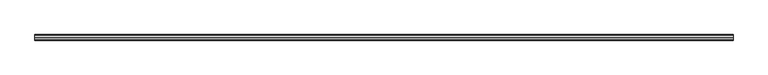
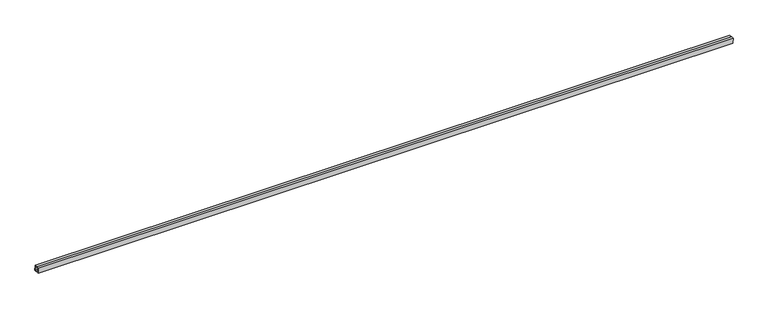
"""IFC4 building model written with IfcOpenShell, lengths in millimetres: proxy geometry, Inner panel:Inner panel:1:Inner panel:1 : Inner panel:Inner panel:300324:2:Inner panel:1:Inner panel:1 : Inner panel:Inner panel:300324:2 : Inner panel:Inner panel:1:Inner panel:1 : Inner panel:Inner panel:300324:300043:43 : Inner panel:Inner panel:1:Inner panel:1 : Inner panel:Inner panel:300324:2:Inner panel:1:Inner panel:1 : Inner panel:Inner panel:300324:2 : Inner panel:Inner panel:1:Inner panel:1 : Inner panel:Inner panel:300324:300043:308120."""

from ifc_helpers import new_model, si_unit, frame, origin, place, context, project, spatial, polyline, outline, extrude, source, transform, mapped, element, save


def generic_models_8f4c7b37(model_context):
    return source(origin(), model_context, "Body", "SweptSolid", [
        extrude(outline(polyline([(-580481.3921913, 3888.2024845), (-580463.1517681, 3888.9625021), (-580461.5656444, 3850.895532), (-580499.6326145, 3849.3094083), (-580501.2187382, 3887.3763783), (-580482.9783151, 3888.136396), (-580482.8791823, 3885.7572103), (-580498.7404199, 3885.0963254), (-580497.3525616, 3851.7877266), (-580464.0439628, 3853.1755849), (-580465.431821, 3886.4841837), (-580481.2930586, 3885.8232988), (-580481.3921913, 3888.2024845)])), frame((607854.1367239, 0.0, 0.0), z_axis=(1.0, 0.0, 0.0), x_axis=(0.0, 1.0, 0.0)), (0.0, 0.0, 1.0), 4876.8),
    ])


if __name__ == "__main__":
    model = new_model("IFC4")
    model_context = context("Model", 3, world=origin())
    ifc_project = project(units=[si_unit("LENGTHUNIT", "METRE", prefix="MILLI")], contexts=[model_context])
    site = spatial("IfcSite", under=ifc_project)
    building = spatial("IfcBuilding", under=site)
    placement = place(None, origin())
    generic_models_shape = generic_models_8f4c7b37(model_context)
    element("IfcBuildingElementProxy", 1, Name="Inner panel:Inner panel:1:Inner panel:1 : Inner panel:Inner panel:300324:2:Inner panel:1:Inner panel:1 : Inner panel:Inner panel:300324:2 : Inner panel:Inner panel:1:Inner panel:1 : Inner panel:Inner panel:300324:300043:43 : Inner panel:Inner panel:1:Inner panel:1 : Inner panel:Inner panel:300324:2:Inner panel:1:Inner panel:1 : Inner panel:Inner panel:300324:2 : Inner panel:Inner panel:1:Inner panel:1 : Inner panel:Inner panel:300324:300043:308120", ObjectType="Inner panel:Inner panel:1:Inner panel:1 : Inner panel:Inner panel:300324:2:Inner panel:1:Inner panel:1 : Inner panel:Inner panel:300324:2 : Inner panel:Inner panel:1:Inner panel:1 : Inner panel:Inner panel:300324:300043:43 : Inner panel:Inner panel:1:Inner panel:1 : Inner panel:Inner panel:300324:2:Inner panel:1:Inner panel:1 : Inner panel:Inner panel:300324:2 : Inner panel:Inner panel:1:Inner panel:1 : Inner panel:Inner panel:300324:300043:308120", at=placement, inside=building, context=model_context, shape_type="MappedRepresentation", body=[
        mapped(generic_models_shape, transform((0.0, 0.0, 0.0), x_axis=(1.0, 0.0, 0.0), y_axis=(0.0, 1.0, 0.0), z_axis=(0.0, 0.0, 1.0))),
    ])
    save(model, "model.ifc")

# Revit data of these elements
# Type "Inner panel:Inner panel:1:Inner panel:1 : Inner panel:Inner panel:300324:2:Inner panel:1:Inner panel:1 : Inner panel:Inner panel:300324:2 : Inner panel:Inner panel:1:Inner panel:1 : Inner panel:Inner panel:300324:300043:43 : Inner panel:Inner panel:1:Inner panel:1 : Inner panel:Inner panel:300324:2:Inner panel:1:Inner panel:1 : Inner panel:Inner panel:300324:2 : Inner panel:Inner panel:1:Inner panel:1 : Inner panel:Inner panel:300324:300043:308120"
#   NameOverride = "Inner panel:Inner panel:1:Inner panel:1 : Inner panel:Inner panel:300324:2:Inner panel:1:Inner panel:1 : Inner panel:Inner panel:300324:2 : Inner panel:Inner panel:1:Inner panel:1 : Inner panel:Inner panel:300324:300043:308120"
#   ObjectTypeOverride = "Inner panel:1:Inner panel:1 : Inner panel:Inner panel:300324:2 : Inner panel:Inner panel:1:Inner panel:1 : Inner panel:Inner panel:300324:300043"
#   Reference = "Inner panel"
#   Tag = "308120"
# Element 1 (IfcBuildingElementProxy, "Inner panel:Inner panel:1:Inner panel:1 : Inner panel:Inner panel:300324:2:Inner panel:1:Inner panel:1 : Inner panel:Inner panel:300324:2 : Inner panel:Inner panel:1:Inner panel:1 : Inner panel:Inner panel:300324:300043:43 : Inner panel:Inner panel:1:Inner panel:1 : Inner panel:Inner panel:300324:2:Inner panel:1:Inner panel:1 : Inner panel:Inner panel:300324:2 : Inner panel:Inner panel:1:Inner panel:1 : Inner panel:Inner panel:300324:300043:308120")
#   Materials on its faces: "1 1/2\" X 1 1/2\" SPLIT-SEAM SQUARE TUBING (~24\" CANTILEVER FROM C.L. OF GLULAM)"
# Materials
#   "1 1/2\" X 1 1/2\" SPLIT-SEAM SQUARE TUBING (~24\" CANTILEVER FROM C.L. OF GLULAM)": class "Unassigned", colour RGB 202 201 200, transparency 0, Cost = 0
